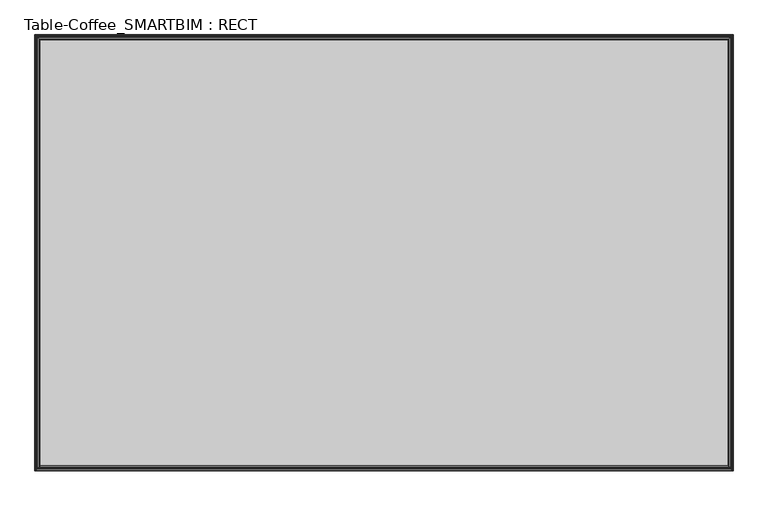
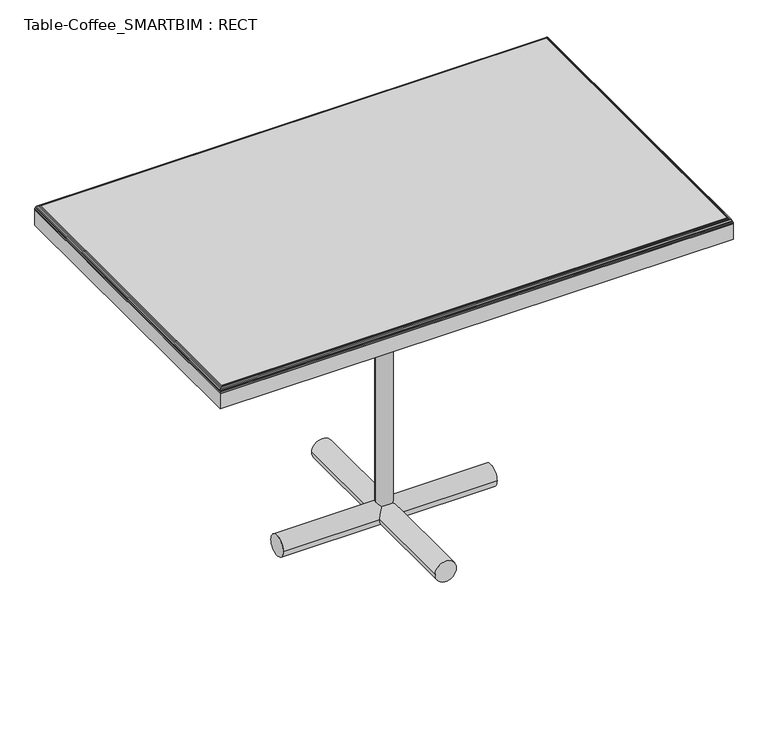
"""IFC4 building model written with IfcOpenShell, lengths in millimetres: furniture geometry, Table-Coffee_SMARTBIM : RECT."""

from ifc_helpers import new_model, si_unit, point, frame, frame_2d, origin, origin_2d, place, context, project, spatial, polyline, circle_curve, ellipse_curve, trimmed, segment, composite_curve, outline, extrude, source, transform, mapped, element, save
from ifc_brep_helpers import plane_surface, cylinder_surface, advanced_brep


def table_coffee_smartbim_rect_01a6e93b(model_context):
    return source(origin(), model_context, "Body", "SolidModel", [
        extrude(outline(composite_curve([segment(trimmed(circle_curve(frame_2d((0.0, 25.4)), 25.4), [point((25.4, 25.4))], [point((-25.4, 25.4))], False, "CARTESIAN"), True, "CONTINUOUS"), segment(trimmed(circle_curve(frame_2d((0.0, 25.4)), 25.4), [point((-25.4, 25.4))], [point((25.4, 25.4))], False, "CARTESIAN"), True, "CONTINUOUS")], self_intersect=False)), frame((-254.0, 0.0, 0.0), z_axis=(1.0, 0.0, 0.0), x_axis=(0.0, 1.0, 0.0)), (0.0, 0.0, 1.0), 508.0),
        extrude(outline(composite_curve([segment(trimmed(circle_curve(frame_2d((25.4, 0.0)), 25.4), [point((25.4, -25.4))], [point((25.4, 25.4))], False, "CARTESIAN"), True, "CONTINUOUS"), segment(trimmed(circle_curve(frame_2d((25.4, 0.0)), 25.4), [point((25.4, 25.4))], [point((25.4, -25.4))], False, "CARTESIAN"), True, "CONTINUOUS")], self_intersect=False)), frame((0.0, -254.0, 0.0), z_axis=(0.0, 1.0, 0.0), x_axis=(0.0, 0.0, 1.0)), (0.0, 0.0, 1.0), 508.0),
        extrude(outline(polyline([(609.6, 381.0), (609.6, -381.0), (-609.6, -381.0), (-609.6, 381.0), (609.6, 381.0)])), frame((0.0, 0.0, 723.9), z_axis=(0.0, 0.0, 1.0), x_axis=(1.0, 0.0, 0.0)), (0.0, 0.0, 1.0), 38.1),
        advanced_brep(
        [(-600.1998654, -371.5998654, 774.7), (600.1998654, -371.5998654, 774.7), (600.1998654, 371.5998654, 774.7), (-600.1998654, 371.5998654, 774.7), (609.6, 381.0, 762.0), (609.6, -381.0, 762.0), (-609.6, -381.0, 762.0), (-609.6, 381.0, 762.0), (-609.6, 381.0, 765.2998654), (609.6, 381.0, 765.2998654), (-609.6, -381.0, 765.2998654), (609.6, -381.0, 765.2998654), (-609.2372483, -380.6372483, 767.8860287), (-609.2372483, 380.6372483, 767.8860287), (-602.3616212, 373.7616212, 774.4480533), (-602.3616212, -373.7616212, 774.4480533), (-604.3639185, 375.7639185, 773.7273912), (-604.3639185, -375.7639185, 773.7273912), (-606.4885738, 377.8885738, 772.2866155), (-606.4885738, -377.8885738, 772.2866155), (-608.5102962, 379.9102962, 769.692959), (-608.5102962, -379.9102962, 769.692959), (609.2372483, -380.6372483, 767.8860287), (602.3616212, -373.7616212, 774.4480533), (604.3639185, -375.7639185, 773.7273912), (606.4885738, -377.8885738, 772.2866155), (608.5102962, -379.9102962, 769.692959), (609.2372483, 380.6372483, 767.8860287), (602.3616212, 373.7616212, 774.4480533), (604.3639185, 375.7639185, 773.7273912), (606.4885738, 377.8885738, 772.2866155), (608.5102962, 379.9102962, 769.692959)],
        [
            (0, 1),
            (1, 2),
            (2, 3),
            (3, 0),
            (4, 5),
            (5, 6),
            (6, 7),
            (7, 4),
            (7, 8),
            (8, 9),
            (9, 4),
            (6, 10),
            (10, 8),
            (5, 11),
            (11, 10),
            (9, 11),
            (10, 12, ellipse_curve(frame((-600.1998654, -371.5998654, 765.2998654), z_axis=(-0.7071067811865475, 0.7071067811865475, 0.0), x_axis=(-0.7071067811865474, -0.7071067811865476, 0.0)), 13.2937978, 9.4001346)),
            (12, 13),
            (13, 8, ellipse_curve(frame((-600.1998654, 371.5998654, 765.2998654), z_axis=(-0.7071067811865475, -0.7071067811865475, 0.0), x_axis=(0.7071067811865474, -0.7071067811865476, 0.0)), 13.2937978, 9.4001346)),
            (14, 15),
            (15, 0, ellipse_curve(frame((-600.1998654, -371.5998654, 765.2998654), z_axis=(-0.7071067811865475, 0.7071067811865475, 0.0), x_axis=(-0.7071067811865474, -0.7071067811865476, 0.0)), 13.2937978, 9.4001346)),
            (3, 14, ellipse_curve(frame((-600.1998654, 371.5998654, 765.2998654), z_axis=(-0.7071067811865475, -0.7071067811865475, 0.0), x_axis=(0.7071067811865474, -0.7071067811865476, 0.0)), 13.2937978, 9.4001346)),
            (14, 16, ellipse_curve(frame((-600.1998654, 371.5998654, 765.2998654), z_axis=(-0.7071067811865475, -0.7071067811865475, 0.0), x_axis=(0.7071067811865474, -0.7071067811865476, 0.0)), 13.2937978, 9.4001346)),
            (16, 17),
            (17, 15, ellipse_curve(frame((-600.1998654, -371.5998654, 765.2998654), z_axis=(-0.7071067811865475, 0.7071067811865475, 0.0), x_axis=(-0.7071067811865474, -0.7071067811865476, 0.0)), 13.2937978, 9.4001346)),
            (16, 18, ellipse_curve(frame((-600.1998654, 371.5998654, 765.2998654), z_axis=(-0.7071067811865475, -0.7071067811865475, 0.0), x_axis=(0.7071067811865474, -0.7071067811865476, 0.0)), 13.2937978, 9.4001346)),
            (18, 19),
            (19, 17, ellipse_curve(frame((-600.1998654, -371.5998654, 765.2998654), z_axis=(-0.7071067811865475, 0.7071067811865475, 0.0), x_axis=(-0.7071067811865474, -0.7071067811865476, 0.0)), 13.2937978, 9.4001346)),
            (18, 20, ellipse_curve(frame((-600.1998654, 371.5998654, 765.2998654), z_axis=(-0.7071067811865475, -0.7071067811865475, 0.0), x_axis=(0.7071067811865474, -0.7071067811865476, 0.0)), 13.2937978, 9.4001346)),
            (20, 21),
            (21, 19, ellipse_curve(frame((-600.1998654, -371.5998654, 765.2998654), z_axis=(-0.7071067811865475, 0.7071067811865475, 0.0), x_axis=(-0.7071067811865474, -0.7071067811865476, 0.0)), 13.2937978, 9.4001346)),
            (12, 21, ellipse_curve(frame((-600.1998654, -371.5998654, 765.2998654), z_axis=(-0.7071067811865475, 0.7071067811865475, 0.0), x_axis=(-0.7071067811865474, -0.7071067811865476, 0.0)), 13.2937978, 9.4001346)),
            (20, 13, ellipse_curve(frame((-600.1998654, 371.5998654, 765.2998654), z_axis=(-0.7071067811865475, -0.7071067811865475, 0.0), x_axis=(0.7071067811865474, -0.7071067811865476, 0.0)), 13.2937978, 9.4001346)),
            (11, 22, ellipse_curve(frame((600.1998654, -371.5998654, 765.2998654), z_axis=(-0.7071067811865475, -0.7071067811865475, 0.0), x_axis=(0.7071067811865476, -0.7071067811865474, 0.0)), 13.2937978, 9.4001346)),
            (22, 12),
            (15, 23),
            (23, 1, ellipse_curve(frame((600.1998654, -371.5998654, 765.2998654), z_axis=(-0.7071067811865475, -0.7071067811865475, 0.0), x_axis=(0.7071067811865476, -0.7071067811865474, 0.0)), 13.2937978, 9.4001346)),
            (17, 24),
            (24, 23, ellipse_curve(frame((600.1998654, -371.5998654, 765.2998654), z_axis=(-0.7071067811865475, -0.7071067811865475, 0.0), x_axis=(0.7071067811865476, -0.7071067811865474, 0.0)), 13.2937978, 9.4001346)),
            (19, 25),
            (25, 24, ellipse_curve(frame((600.1998654, -371.5998654, 765.2998654), z_axis=(-0.7071067811865475, -0.7071067811865475, 0.0), x_axis=(0.7071067811865476, -0.7071067811865474, 0.0)), 13.2937978, 9.4001346)),
            (21, 26),
            (26, 25, ellipse_curve(frame((600.1998654, -371.5998654, 765.2998654), z_axis=(-0.7071067811865475, -0.7071067811865475, 0.0), x_axis=(0.7071067811865476, -0.7071067811865474, 0.0)), 13.2937978, 9.4001346)),
            (22, 26, ellipse_curve(frame((600.1998654, -371.5998654, 765.2998654), z_axis=(-0.7071067811865475, -0.7071067811865475, 0.0), x_axis=(0.7071067811865476, -0.7071067811865474, 0.0)), 13.2937978, 9.4001346)),
            (9, 27, ellipse_curve(frame((600.1998654, 371.5998654, 765.2998654), z_axis=(0.7071067811865475, -0.7071067811865475, 0.0), x_axis=(0.7071067811865474, 0.7071067811865476, 0.0)), 13.2937978, 9.4001346)),
            (27, 22),
            (23, 28),
            (28, 2, ellipse_curve(frame((600.1998654, 371.5998654, 765.2998654), z_axis=(0.7071067811865475, -0.7071067811865475, 0.0), x_axis=(0.7071067811865474, 0.7071067811865476, 0.0)), 13.2937978, 9.4001346)),
            (24, 29),
            (29, 28, ellipse_curve(frame((600.1998654, 371.5998654, 765.2998654), z_axis=(0.7071067811865475, -0.7071067811865475, 0.0), x_axis=(0.7071067811865474, 0.7071067811865476, 0.0)), 13.2937978, 9.4001346)),
            (25, 30),
            (30, 29, ellipse_curve(frame((600.1998654, 371.5998654, 765.2998654), z_axis=(0.7071067811865475, -0.7071067811865475, 0.0), x_axis=(0.7071067811865474, 0.7071067811865476, 0.0)), 13.2937978, 9.4001346)),
            (26, 31),
            (31, 30, ellipse_curve(frame((600.1998654, 371.5998654, 765.2998654), z_axis=(0.7071067811865475, -0.7071067811865475, 0.0), x_axis=(0.7071067811865474, 0.7071067811865476, 0.0)), 13.2937978, 9.4001346)),
            (27, 31, ellipse_curve(frame((600.1998654, 371.5998654, 765.2998654), z_axis=(0.7071067811865475, -0.7071067811865475, 0.0), x_axis=(0.7071067811865474, 0.7071067811865476, 0.0)), 13.2937978, 9.4001346)),
            (13, 27),
            (28, 14),
            (29, 16),
            (30, 18),
            (31, 20),
        ],
        [
            plane_surface(frame((-609.6, 381.0, 774.7), z_axis=(0.0, 0.0, 1.0), x_axis=(-1.0, 0.0, 0.0))),
            plane_surface(frame((-609.6, 381.0, 762.0), z_axis=(0.0, 0.0, -1.0), x_axis=(1.0, 0.0, 0.0))),
            plane_surface(frame((609.6, 381.0, 774.7), z_axis=(0.0, 1.0, 0.0), x_axis=(0.0, 0.0, -1.0))),
            plane_surface(frame((-609.6, 381.0, 774.7), z_axis=(-1.0, 0.0, 0.0), x_axis=(0.0, 0.0, -1.0))),
            plane_surface(frame((-609.6, -381.0, 774.7), z_axis=(0.0, -1.0, 0.0), x_axis=(0.0, 0.0, -1.0))),
            plane_surface(frame((609.6, -381.0, 774.7), z_axis=(1.0, 0.0, 0.0), x_axis=(0.0, 0.0, -1.0))),
            cylinder_surface(frame((-600.1998654, 381.0, 765.2998654), z_axis=(0.0, -1.0, 0.0), x_axis=(1.0, 0.0, 0.0)), 9.4001346),
            cylinder_surface(frame((-609.6, -371.5998654, 765.2998654), z_axis=(1.0, 0.0, 0.0), x_axis=(0.0, 1.0, 0.0)), 9.4001346),
            cylinder_surface(frame((600.1998654, -381.0, 765.2998654), z_axis=(0.0, 1.0, 0.0), x_axis=(-1.0, 0.0, 0.0)), 9.4001346),
            cylinder_surface(frame((609.6, 371.5998654, 765.2998654), z_axis=(-1.0, 0.0, 0.0), x_axis=(0.0, -1.0, 0.0)), 9.4001346),
        ],
        [
            (0, [[1, 2, 3, 4]]),
            (1, [[5, 6, 7, 8]]),
            (2, [[-8, 9, 10, 11]]),
            (3, [[-7, 12, 13, -9]]),
            (4, [[-6, 14, 15, -12]]),
            (5, [[-5, -11, 16, -14]]),
            (6, [[17, 18, 19, -13]]),
            (6, [[20, 21, -4, 22]]),
            (6, [[-20, 23, 24, 25]]),
            (6, [[-24, 26, 27, 28]]),
            (6, [[-27, 29, 30, 31]]),
            (6, [[-18, 32, -30, 33]]),
            (7, [[-17, -15, 34, 35]]),
            (7, [[-21, 36, 37, -1]]),
            (7, [[-25, 38, 39, -36]]),
            (7, [[-28, 40, 41, -38]]),
            (7, [[-31, 42, 43, -40]]),
            (7, [[-32, -35, 44, -42]]),
            (8, [[-34, -16, 45, 46]]),
            (8, [[-37, 47, 48, -2]]),
            (8, [[-39, 49, 50, -47]]),
            (8, [[-41, 51, 52, -49]]),
            (8, [[-43, 53, 54, -51]]),
            (8, [[-44, -46, 55, -53]]),
            (9, [[-19, 56, -45, -10]]),
            (9, [[-22, -3, -48, 57]]),
            (9, [[-23, -57, -50, 58]]),
            (9, [[-26, -58, -52, 59]]),
            (9, [[-29, -59, -54, 60]]),
            (9, [[-33, -60, -55, -56]]),
        ],
    ),
        extrude(outline(polyline([(76.2, 76.2), (76.2, -76.2), (-76.2, -76.2), (-76.2, 76.2), (76.2, 76.2)])), frame((0.0, 0.0, 755.65), z_axis=(0.0, 0.0, 1.0), x_axis=(1.0, 0.0, 0.0)), (0.0, 0.0, 1.0), 6.35),
        extrude(outline(composite_curve([segment(trimmed(circle_curve(origin_2d(), 19.05), [point((-19.05, 0.0))], [point((19.05, 0.0))], False, "CARTESIAN"), True, "CONTINUOUS"), segment(trimmed(circle_curve(origin_2d(), 19.05), [point((19.05, 0.0))], [point((-19.05, 0.0))], False, "CARTESIAN"), True, "CONTINUOUS")], self_intersect=False)), frame((0.0, 0.0, 24.2070278), z_axis=(0.0, 0.0, 1.0), x_axis=(1.0, 0.0, 0.0)), (0.0, 0.0, 1.0), 731.4429722),
    ])


if __name__ == "__main__":
    model = new_model("IFC4")
    model_context = context("Model", 3, world=origin())
    ifc_project = project(units=[si_unit("LENGTHUNIT", "METRE", prefix="MILLI")], contexts=[model_context])
    site = spatial("IfcSite", under=ifc_project)
    building = spatial("IfcBuilding", under=site)
    placement = place(None, origin())
    table_coffee_smartbim_rect_shape = table_coffee_smartbim_rect_01a6e93b(model_context)
    element("IfcFurniture", 1, ObjectType="Table-Coffee_SMARTBIM : RECT", at=placement, inside=building, context=model_context, shape_type="MappedRepresentation", body=[
        mapped(table_coffee_smartbim_rect_shape, transform((0.0, 0.0, 0.0), x_axis=(1.0, 0.0, 0.0), y_axis=(0.0, 1.0, 0.0), z_axis=(0.0, 0.0, 1.0))),
    ])
    save(model, "model.ifc")

# Revit data of these elements
# Project information
#   Project Issue Date = "05/20/2019"
#   Project Status = "Project Status"
#   Client Name = "Owner"
#   Project Address = "SOMERS, WI"
#   Project Name = "OAKFIRE 2.0"
#   Project Number = "Project Number"
# Type "Table-Coffee_SMARTBIM : RECT"
#   Subcategory = "Table\r\n"
#   SmartBIM Object Created By = "SMARTBIM, LLC"
#   Manufacturer = "SMARTBIM"
#   Assembly Code = "E2020200"
#   95 CSI = "12500"
#   04 CSI = "12 50 00"
#   table cloth = 0' - 1 1/2"
#   Width = 4' - 0"
#   SmartBIM Object Version = 3
#   Height = 2' - 6"
#   Depth = 2' - 6"
#   Default Elevation = 4' - 0"
#   white cloth_parameter = WOOD-OAKFIRE
#   Table Unit = MET
#   Glide = none
#   Glass = none
# Element 1 (IfcFurniture, "Table-Coffee_SMARTBIM : RECT")
#   Materials on its faces: "WOOD-OAKFIRE", "MET"
# Materials
#   "WOOD-OAKFIRE": class "Wood", colour RGB 198 202 183, transparency 0, Description = "Generic wood", Cost = 0
#   "MET": class "Metal", colour RGB 189 187 185, transparency 0
